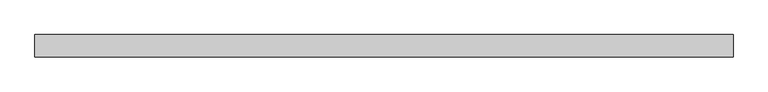
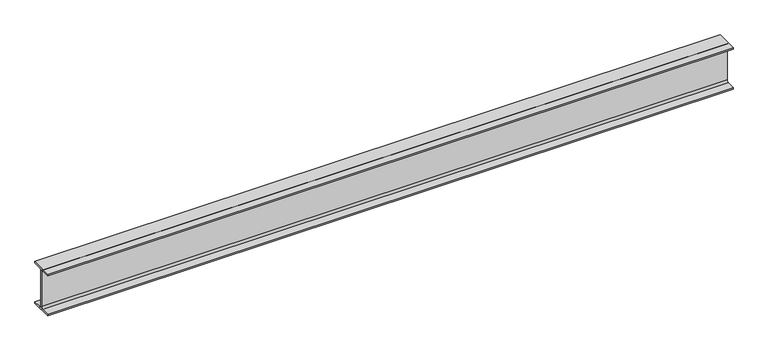
"""IFC4 building model written with IfcOpenShell, lengths in millimetres: beam geometry, 0912_Steel Framing_H-KSD3502 : H_SB_ASB_H-250x125x6x9."""

from ifc_helpers import new_model, si_unit, point, frame, frame_2d, origin, place, context, project, spatial, polyline, circle_curve, trimmed, segment, composite_curve, outline, extrude, source, transform, mapped, element, save


def beam_1ee0d709(model_context):
    return source(origin(), model_context, "Body", "SweptSolid", [
        extrude(outline(composite_curve([segment(polyline([(62.5, -116.0), (62.5, -125.0), (-62.5, -125.0), (-62.5, -116.0), (-15.0, -116.0)]), True, "CONTINUOUS"), segment(trimmed(circle_curve(frame_2d((-15.0, -104.0)), 12.0), [point((-15.0, -116.0))], [point((-3.0, -104.0))], True, "CARTESIAN"), True, "CONTINUOUS"), segment(polyline([(-3.0, -104.0), (-3.0, 104.0)]), True, "CONTINUOUS"), segment(trimmed(circle_curve(frame_2d((-15.0, 104.0)), 12.0), [point((-3.0, 104.0))], [point((-15.0, 116.0))], True, "CARTESIAN"), True, "CONTINUOUS"), segment(polyline([(-15.0, 116.0), (-62.5, 116.0), (-62.5, 125.0), (62.5, 125.0), (62.5, 116.0), (15.0, 116.0)]), True, "CONTINUOUS"), segment(trimmed(circle_curve(frame_2d((15.0, 104.0)), 12.0), [point((15.0, 116.0))], [point((3.0, 104.0))], True, "CARTESIAN"), True, "CONTINUOUS"), segment(polyline([(3.0, 104.0), (3.0, -104.0)]), True, "CONTINUOUS"), segment(trimmed(circle_curve(frame_2d((15.0, -104.0)), 12.0), [point((3.0, -104.0))], [point((15.0, -116.0))], True, "CARTESIAN"), True, "CONTINUOUS"), segment(polyline([(15.0, -116.0), (62.5, -116.0)]), True, "CONTINUOUS")], self_intersect=False)), frame((-1904.8, 0.0, 0.0), z_axis=(1.0, 0.0, 0.0), x_axis=(0.0, 1.0, 0.0)), (0.0, 0.0, 1.0), 3892.0999994),
    ])


if __name__ == "__main__":
    model = new_model("IFC4")
    model_context = context("Model", 3, world=origin())
    ifc_project = project(units=[si_unit("LENGTHUNIT", "METRE", prefix="MILLI")], contexts=[model_context])
    site = spatial("IfcSite", under=ifc_project)
    building = spatial("IfcBuilding", under=site)
    placement = place(None, origin())
    beam_shape = beam_1ee0d709(model_context)
    element("IfcBeam", 1, ObjectType="0912_Steel Framing_H-KSD3502 : H_SB_ASB_H-250x125x6x9", at=placement, inside=building, context=model_context, shape_type="MappedRepresentation", body=[
        mapped(beam_shape, transform((0.0, 0.0, 0.0), x_axis=(1.0, 0.0, 0.0), y_axis=(0.0, 1.0, 0.0), z_axis=(0.0, 0.0, 1.0))),
    ])
    save(model, "model.ifc")

# Revit data of these elements
# Type "0912_Steel Framing_H-KSD3502 : H_SB_ASB_H-250x125x6x9"
#   H_WM Code_1 = "S01AA003-00001 | Main Steel Structure Fabrication Work | Shelter/Building | Light Steel - Standard (30KG/M>Weight) | Material: (   )"
#   H_WM Code_2 = "S03AA029-00001 | Main Steel Structure Erection Work | Shelter/Building | Light Steel (30KG/M>Weight) | Material: (   )"
#   H_WM Code_3 = "S01AA010-00001 | Main Steel Structure Fabrication Work | Shelter/Building | Steel Painting/Coating | for Non-Fireproofed Steel Surface, Surface Preparation, Primer, Second & Final Coat | Material: (   )"
#   H_Q'ty Cal Type Tag = "SB-Q2"
#   Width = 12.5 cm
#   Web Thickness = 0.6 cm
#   Web Fillet = 1.2 cm
#   Warping Constant = 42539.8 cm⁶
#   W = 0
#   Torsional Moment of Inertia = 7.8102 cm⁴
#   Section Area = 37.66 cm²
#   Plastic Modulus weak axis = 73.1 cm³
#   Plastic Modulus strong axis = 366.0 cm³
#   Perimeter = 0.97 m²/m
#   Nominal Weight = 29.60 kgf/m
#   Moment of Inertia weak axis = 294.00 cm⁴
#   Moment of Inertia strong axis = 4050.00 cm⁴
#   Height = 25.0 cm
#   Flange Thickness = 0.9 cm
#   Elastic Modulus weak axis = 47.0 cm³
#   Elastic Modulus strong axis = 324.0 cm³
#   Centroid Vertical = 12.5 cm
#   Centroid Horizontal = 6.25 cm
#   Ix = 40500000
#   Length [instance default] = 1.5240 m
#   Zx = 366000
#   b = 0.1250 m
#   h = 0.2500 m
#   r = 0.0120 m
#   s = 0.0060 m
#   t = 0.0090 m
#   A = 0.003766 m²
#   Structural Material [instance default] = Steel, 45-345
#   Assembly Code = ""
# Element 1 (IfcBeam, "0912_Steel Framing_H-KSD3502 : H_SB_ASB_H-250x125x6x9")
#   Structural Material = none
# Materials
#   "Steel, 45-345": class "Metal", colour RGB 189 187 185, transparency 0, Description = "Steel 345 MPa", Cost = 0
